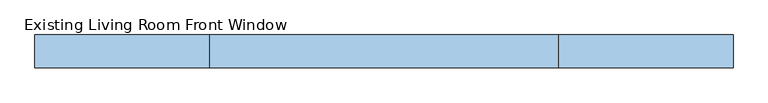
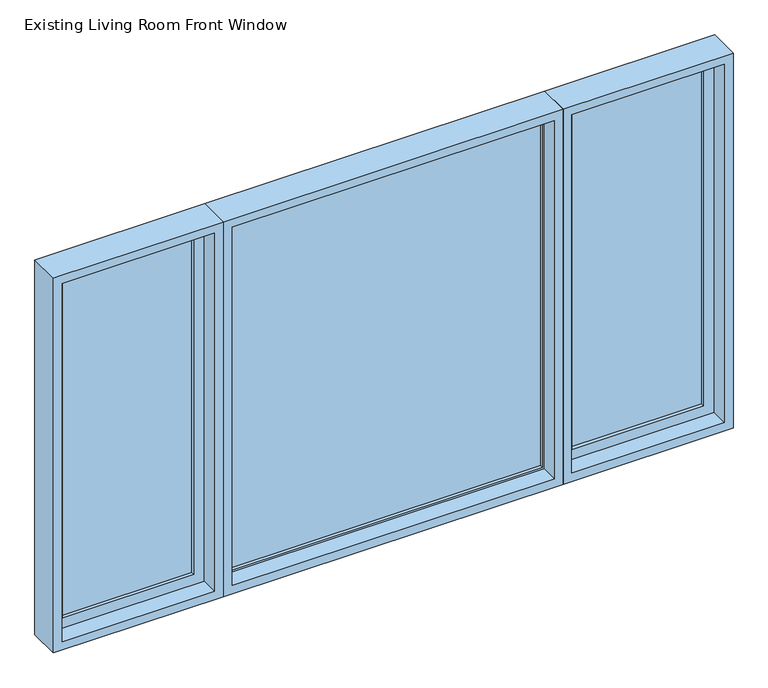
"""IFC4 building model written with IfcOpenShell, lengths in millimetres: window geometry, Existing Living Room Front Window."""

from ifc_helpers import new_model, si_unit, frame, origin, place, context, project, spatial, polyline, outline, extrude, faceted_brep, source, transform, mapped, element, save


def existing_living_room_front_window_c9edc87e(model_context):
    return source(origin(), model_context, "Body", "SolidModel", [
        extrude(outline(polyline([(-1149.35, 176.2125), (-679.45, 176.2125), (-679.45, 169.8625), (-1149.35, 169.8625), (-1149.35, 176.2125)])), frame((0.0, 0.0, 984.25), z_axis=(0.0, 0.0, 1.0), x_axis=(1.0, 0.0, 0.0)), (0.0, 0.0, 1.0), 1282.7),
        extrude(outline(polyline([(-679.45, 157.1625), (-1149.35, 157.1625), (-1149.35, 163.5125), (-679.45, 163.5125), (-679.45, 157.1625)])), frame((0.0, 0.0, 984.25), z_axis=(0.0, 0.0, 1.0), x_axis=(1.0, 0.0, 0.0)), (0.0, 0.0, 1.0), 1282.7),
        extrude(outline(polyline([(2324.1, -622.3), (2324.1, -1206.5), (927.1, -1206.5), (927.1, -622.3), (2324.1, -622.3)]), holes=[polyline([(2266.95, -1149.35), (2266.95, -679.45), (984.25, -679.45), (984.25, -1149.35), (2266.95, -1149.35)])]), frame((0.0, 144.4625, 0.0), z_axis=(0.0, 1.0, 0.0), x_axis=(0.0, 0.0, 1.0)), (0.0, 0.0, 1.0), 44.45),
        faceted_brep([(-1187.45, 144.4625, 2305.05), (-641.35, 144.4625, 2305.05), (-641.35, 80.9625, 2305.05), (-1187.45, 80.9625, 2305.05), (-1206.5, 195.2625, 2324.1), (-622.3, 195.2625, 2324.1), (-622.3, 144.4625, 2324.1), (-1206.5, 144.4625, 2324.1), (-1219.2, 80.9625, 2336.8), (-609.6, 80.9625, 2336.8), (-609.6, 195.2625, 2336.8), (-1219.2, 195.2625, 2336.8), (-641.35, 144.4625, 946.15), (-641.35, 80.9625, 946.15), (-622.3, 195.2625, 927.1), (-622.3, 144.4625, 927.1), (-609.6, 80.9625, 914.4), (-609.6, 195.2625, 914.4), (-1187.45, 144.4625, 946.15), (-1187.45, 80.9625, 946.15), (-1206.5, 195.2625, 927.1), (-1206.5, 144.4625, 927.1), (-1219.2, 80.9625, 914.4), (-1219.2, 195.2625, 914.4)], [[[0, 1, 2, 3]], [[4, 5, 6, 7]], [[8, 9, 10, 11]], [[1, 12, 13, 2]], [[5, 14, 15, 6]], [[9, 16, 17, 10]], [[12, 18, 19, 13]], [[14, 20, 21, 15]], [[16, 22, 23, 17]], [[9, 8, 22, 16], [3, 2, 13, 19]], [[18, 0, 3, 19]], [[7, 6, 15, 21], [1, 0, 18, 12]], [[20, 4, 7, 21]], [[22, 8, 11, 23]], [[11, 10, 17, 23], [5, 4, 20, 14]]]),
        extrude(outline(polyline([(679.45, 176.2125), (1149.35, 176.2125), (1149.35, 169.8625), (679.45, 169.8625), (679.45, 176.2125)])), frame((0.0, 0.0, 984.25), z_axis=(0.0, 0.0, 1.0), x_axis=(1.0, 0.0, 0.0)), (0.0, 0.0, 1.0), 1282.7),
        extrude(outline(polyline([(1149.35, 157.1625), (679.45, 157.1625), (679.45, 163.5125), (1149.35, 163.5125), (1149.35, 157.1625)])), frame((0.0, 0.0, 984.25), z_axis=(0.0, 0.0, 1.0), x_axis=(1.0, 0.0, 0.0)), (0.0, 0.0, 1.0), 1282.7),
        extrude(outline(polyline([(2324.1, 1206.5), (2324.1, 622.3), (927.1, 622.3), (927.1, 1206.5), (2324.1, 1206.5)]), holes=[polyline([(2266.95, 679.45), (2266.95, 1149.35), (984.25, 1149.35), (984.25, 679.45), (2266.95, 679.45)])]), frame((0.0, 144.4625, 0.0), z_axis=(0.0, 1.0, 0.0), x_axis=(0.0, 0.0, 1.0)), (0.0, 0.0, 1.0), 44.45),
        faceted_brep([(641.35, 144.4625, 2305.05), (1187.45, 144.4625, 2305.05), (1187.45, 80.9625, 2305.05), (641.35, 80.9625, 2305.05), (622.3, 195.2625, 2324.1), (1206.5, 195.2625, 2324.1), (1206.5, 144.4625, 2324.1), (622.3, 144.4625, 2324.1), (609.6, 80.9625, 2336.8), (1219.2, 80.9625, 2336.8), (1219.2, 195.2625, 2336.8), (609.6, 195.2625, 2336.8), (1187.45, 144.4625, 946.15), (1187.45, 80.9625, 946.15), (1206.5, 195.2625, 927.1), (1206.5, 144.4625, 927.1), (1219.2, 80.9625, 914.4), (1219.2, 195.2625, 914.4), (641.35, 144.4625, 946.15), (641.35, 80.9625, 946.15), (622.3, 195.2625, 927.1), (622.3, 144.4625, 927.1), (609.6, 80.9625, 914.4), (609.6, 195.2625, 914.4)], [[[0, 1, 2, 3]], [[4, 5, 6, 7]], [[8, 9, 10, 11]], [[1, 12, 13, 2]], [[5, 14, 15, 6]], [[9, 16, 17, 10]], [[12, 18, 19, 13]], [[14, 20, 21, 15]], [[16, 22, 23, 17]], [[9, 8, 22, 16], [3, 2, 13, 19]], [[18, 0, 3, 19]], [[7, 6, 15, 21], [1, 0, 18, 12]], [[20, 4, 7, 21]], [[22, 8, 11, 23]], [[11, 10, 17, 23], [5, 4, 20, 14]]]),
        extrude(outline(polyline([(-571.5, 176.2125), (571.5, 176.2125), (571.5, 169.8625), (-571.5, 169.8625), (-571.5, 176.2125)])), frame((0.0, 0.0, 952.5), z_axis=(0.0, 0.0, 1.0), x_axis=(1.0, 0.0, 0.0)), (0.0, 0.0, 1.0), 1346.2),
        extrude(outline(polyline([(571.5, 157.1625), (-571.5, 157.1625), (-571.5, 163.5125), (571.5, 163.5125), (571.5, 157.1625)])), frame((0.0, 0.0, 952.5), z_axis=(0.0, 0.0, 1.0), x_axis=(1.0, 0.0, 0.0)), (0.0, 0.0, 1.0), 1346.2),
        extrude(outline(polyline([(927.1, -596.9), (927.1, 596.9), (2324.1, 596.9), (2324.1, -596.9), (927.1, -596.9)]), holes=[polyline([(952.5, 571.5), (952.5, -571.5), (2298.7, -571.5), (2298.7, 571.5), (952.5, 571.5)])]), frame((0.0, 144.4625, 0.0), z_axis=(0.0, 1.0, 0.0), x_axis=(0.0, 0.0, 1.0)), (0.0, 0.0, 1.0), 44.45),
        faceted_brep([(-609.6, 80.9625, 2336.8), (609.6, 80.9625, 2336.8), (609.6, 195.2625, 2336.8), (-609.6, 195.2625, 2336.8), (609.6, 80.9625, 914.4), (609.6, 195.2625, 914.4), (-609.6, 80.9625, 914.4), (-609.6, 195.2625, 914.4), (-577.85, 80.9625, 2305.05), (577.85, 80.9625, 2305.05), (577.85, 80.9625, 946.15), (-577.85, 80.9625, 946.15), (596.9, 195.2625, 2324.1), (-596.9, 195.2625, 2324.1), (-596.9, 195.2625, 927.1), (596.9, 195.2625, 927.1), (-577.85, 144.4625, 2305.05), (577.85, 144.4625, 2305.05), (596.9, 144.4625, 2324.1), (-596.9, 144.4625, 2324.1), (577.85, 144.4625, 946.15), (596.9, 144.4625, 927.1), (-577.85, 144.4625, 946.15), (-596.9, 144.4625, 927.1)], [[[0, 1, 2, 3]], [[1, 4, 5, 2]], [[4, 6, 7, 5]], [[1, 0, 6, 4], [8, 9, 10, 11]], [[6, 0, 3, 7]], [[3, 2, 5, 7], [12, 13, 14, 15]], [[16, 17, 9, 8]], [[13, 12, 18, 19]], [[17, 20, 10, 9]], [[12, 15, 21, 18]], [[20, 22, 11, 10]], [[15, 14, 23, 21]], [[22, 16, 8, 11]], [[19, 18, 21, 23], [17, 16, 22, 20]], [[14, 13, 19, 23]]]),
    ])


if __name__ == "__main__":
    model = new_model("IFC4")
    model_context = context("Model", 3, world=origin())
    ifc_project = project(units=[si_unit("LENGTHUNIT", "METRE", prefix="MILLI")], contexts=[model_context])
    site = spatial("IfcSite", under=ifc_project)
    building = spatial("IfcBuilding", under=site)
    placement = place(None, origin())
    existing_living_room_front_window_shape = existing_living_room_front_window_c9edc87e(model_context)
    element("IfcWindow", 1, ObjectType="Existing Living Room Front Window : (2) 2'-0\" x 4'-8\" CS + 4'-0\" x 4'-8\" FX", at=placement, inside=building, context=model_context, shape_type="MappedRepresentation", body=[
        mapped(existing_living_room_front_window_shape, transform((0.0, 0.0, 0.0), x_axis=(1.0, 0.0, 0.0), y_axis=(0.0, 1.0, 0.0), z_axis=(0.0, 0.0, 1.0))),
    ])
    save(model, "model.ifc")

# Revit data of these elements
# Type "Existing Living Room Front Window : (2) 2'-0\" x 4'-8\" CS + 4'-0\" x 4'-8\" FX"
#   Type Mark = "31"
#   Analytic Construction = "<None>"
#   Window Inset = 0' - 0 3/4"
#   Side Window Width = 2' - 0"
#   Side Window Location = 2' - 0"
#   Middle Window Width = 4' - 0"
#   Height = 4' - 8"
#   Default Sill Height = 3' - 0"
#   Width = 8' - 0"
#   Top Muntin Visibility = yes
#   Side Window Nested Trim Visibility = no
#   Interior Trim Visibility [instance default] = yes
#   Fixed Muntin Visibility = no
#   Exterior Trim Visibility [instance default] = yes
#   Define Thermal Properties by = 1
#   Bottom Muntin Visibility = yes
#   Sash Material = Sash
#   Right Side Window Type = element 472099
#   Left Side Window Type = element 472100
#   Interior Trim = Trim-Window-Interior-Flat : Picture Frame
#   Interior Trim Material = Wood - Stained
#   Interior Frame Material = Wood - Stained
#   Glass Pane Material = Glass
#   Exterior Trim Material = Clad - White
#   Exterior Trim = Trim-Window-Exterior-Flat : with Sill
#   Exterior Frame Material = Clad - White
#   Rough Width = 0
#   Rough Height = 0
#   Wall Closure = (empty or 0)
# Element 1 (IfcWindow, "Existing Living Room Front Window : (2) 2'-0\" x 4'-8\" CS + 4'-0\" x 4'-8\" FX")
#   Materials on its faces: "Wood - Stained", "Glass", "Clad - White"
# Materials
#   "Sash": class "Wood", colour RGB 224 178 126, transparency 0, Cost = 0
#   "Wood - Stained": class "Wood", colour RGB 224 178 126, transparency 0, Cost = 0
#   "Glass": class "Glass", colour RGB 0 128 192, transparency 0.75, Description = "Soda Lime Glass", Cost = 0
#   "Clad - White": class "Wood", colour RGB 242 242 238, transparency 0, Cost = 0
